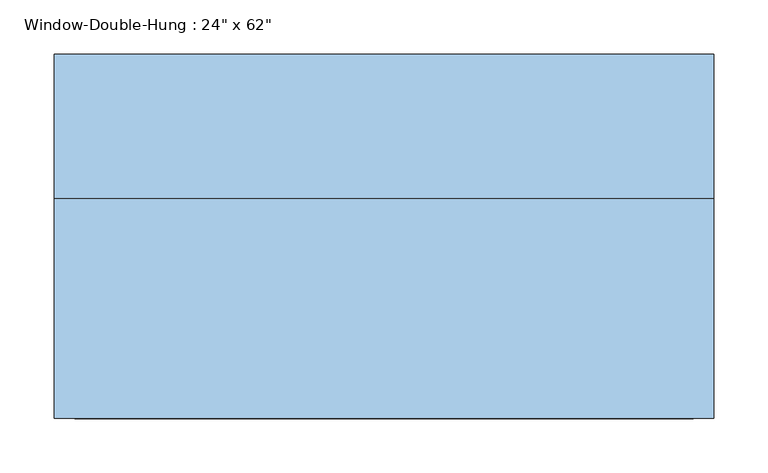
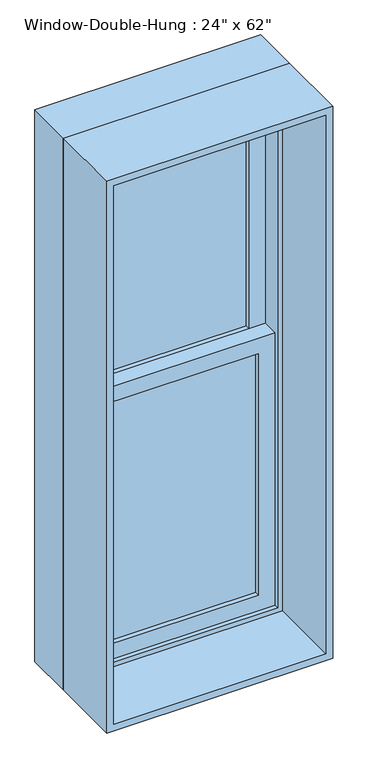
"""IFC4 building model written with IfcOpenShell, lengths in millimetres: window geometry."""

from ifc_helpers import new_model, si_unit, frame, origin, place, context, project, spatial, polyline, outline, extrude, source, transform, mapped, element, save


def window_aa90209f(model_context):
    return source(origin(), model_context, "Body", "SweptSolid", [
        extrude(outline(polyline([(228.6, 88.9), (228.6, 82.55), (-228.6, 82.55), (-228.6, 88.9), (228.6, 88.9)])), frame((0.0, 0.0, 990.6), z_axis=(0.0, 0.0, 1.0), x_axis=(1.0, 0.0, 0.0)), (0.0, 0.0, 1.0), 688.975),
        extrude(outline(polyline([(-228.6, 76.2), (228.6, 76.2), (228.6, 69.85), (-228.6, 69.85), (-228.6, 76.2)])), frame((0.0, 0.0, 990.6), z_axis=(0.0, 0.0, 1.0), x_axis=(1.0, 0.0, 0.0)), (0.0, 0.0, 1.0), 688.975),
        extrude(outline(polyline([(228.6, 133.35), (228.6, 127.0), (-228.6, 127.0), (-228.6, 133.35), (228.6, 133.35)])), frame((0.0, 0.0, 1724.025), z_axis=(0.0, 0.0, 1.0), x_axis=(1.0, 0.0, 0.0)), (0.0, 0.0, 1.0), 688.975),
        extrude(outline(polyline([(-228.6, 120.65), (228.6, 120.65), (228.6, 114.3), (-228.6, 114.3), (-228.6, 120.65)])), frame((0.0, 0.0, 1724.025), z_axis=(0.0, 0.0, 1.0), x_axis=(1.0, 0.0, 0.0)), (0.0, 0.0, 1.0), 688.975),
        extrude(outline(polyline([(1724.025, -273.05), (946.15, -273.05), (946.15, 273.05), (1724.025, 273.05), (1724.025, -273.05)]), holes=[polyline([(1679.575, 228.6), (990.6, 228.6), (990.6, -228.6), (1679.575, -228.6), (1679.575, 228.6)])]), frame((0.0, 57.15, 0.0), z_axis=(0.0, 1.0, 0.0), x_axis=(0.0, 0.0, 1.0)), (0.0, 0.0, 1.0), 44.45),
        extrude(outline(polyline([(2457.45, -273.05), (1679.575, -273.05), (1679.575, 273.05), (2457.45, 273.05), (2457.45, -273.05)]), holes=[polyline([(2413.0, 228.6), (1724.025, 228.6), (1724.025, -228.6), (2413.0, -228.6), (2413.0, 228.6)])]), frame((0.0, 101.6, 0.0), z_axis=(0.0, 1.0, 0.0), x_axis=(0.0, 0.0, 1.0)), (0.0, 0.0, 1.0), 44.45),
        extrude(outline(polyline([(2489.2, -304.8), (914.4, -304.8), (914.4, 304.8), (2489.2, 304.8), (2489.2, -304.8)]), holes=[polyline([(2457.45, 273.05), (946.15, 273.05), (946.15, -273.05), (2457.45, -273.05), (2457.45, 273.05)])]), frame((0.0, 44.45, 0.0), z_axis=(0.0, 1.0, 0.0), x_axis=(0.0, 0.0, 1.0)), (0.0, 0.0, 1.0), 133.35),
        extrude(outline(polyline([(2489.2, 304.8), (2489.2, -304.8), (914.4, -304.8), (914.4, 304.8), (2489.2, 304.8)]), holes=[polyline([(2470.15, 285.75), (933.45, 285.75), (933.45, -285.75), (2470.15, -285.75), (2470.15, 285.75)])]), frame((0.0, -158.75, 0.0), z_axis=(0.0, 1.0, 0.0), x_axis=(0.0, 0.0, 1.0)), (0.0, 0.0, 1.0), 203.2),
    ])


if __name__ == "__main__":
    model = new_model("IFC4")
    model_context = context("Model", 3, world=origin())
    ifc_project = project(units=[si_unit("LENGTHUNIT", "METRE", prefix="MILLI")], contexts=[model_context])
    site = spatial("IfcSite", under=ifc_project)
    building = spatial("IfcBuilding", under=site)
    placement = place(None, origin())
    window_shape = window_aa90209f(model_context)
    element("IfcWindow", 1, ObjectType="Window-Double-Hung : 24\" x 62\"", at=placement, inside=building, context=model_context, shape_type="MappedRepresentation", body=[
        mapped(window_shape, transform((0.0, 0.0, 0.0), x_axis=(1.0, 0.0, 0.0), y_axis=(0.0, 1.0, 0.0), z_axis=(0.0, 0.0, 1.0))),
    ])
    save(model, "model.ifc")

# Revit data of these elements
# Type "Window-Double-Hung : 24\" x 62\""
#   Type Mark = "30"
#   Fire Rating = "0.5h"
#   Construction Type Id = "DG-DR"
#   Assembly Code = "B2020100"
#   Analytic Construction = "Double glazing - domestic"
#   Wall Thickness [instance default] = 0' - 6"
#   Window Inset [instance default] = 0' - 0"
#   Visual Light Transmittance = 0.81
#   Thermal Resistance (R) = 1.8146 (h·ft²·°F)/BTU
#   Solar Heat Gain Coefficient = 0.76
#   Muntin Width = 1' - 6"
#   Muntin Height = 2' - 3 1/8"
#   Interior Wall Closure [instance default] = 0' - 1 1/2"
#   Rough Width = 2' - 0 1/2"
#   Rough Height = 5' - 2 1/2"
#   Frame Extension [instance default] = 0' - 1 1/4"
#   Exterior Wall Closure [instance default] = 0' - 0 1/2"
#   Extension Jamb [instance default] = 0' - 1 1/2"
#   Heat Transfer Coefficient (U) = 0.5511 BTU/(h·ft²·°F)
#   Height = 5' - 2"
#   Width = 2' - 0"
#   Top Muntin Visibility = yes
#   Indicator Visibility [instance default] = yes
#   Extension Jamb Visibility [instance default] = yes
#   Interior Trim Visibility [instance default] = yes
#   Exterior Trim Visibility [instance default] = yes
#   Define Thermal Properties by = 1
#   Bottom Muntin Visibility = yes
#   Muntin Pattern = Muntin Pattern_2x2 : Muntin Pattern_2x2
#   Interior Trim Material = Wood - Stained
#   Interior Trim = Trim-Window-Interior-Flat : Picture Frame
#   Exterior Trim Material = Clad - White
#   Exterior Trim = Trim-Window-Exterior-Flat : with Sill
#   Glass Panel Material = Glass
#   Exterior Frame Material = Clad - White
#   Interior Frame Material = Wood - Stained
#   Wall Closure = (empty or 0)
# Element 1 (IfcWindow, "Window-Double-Hung : 24\" x 62\"")
#   Wall Thickness = 1' - 0 1/2"
#   Extension Jamb = 0' - 8"
#   Materials on its faces: "Wood - Stained", "Glass", "Clad - White"
# Materials
#   "Wood - Stained": class "Wood", colour RGB 224 178 126, transparency 0, Cost = 0
#   "Clad - White": class "Wood", colour RGB 242 242 238, transparency 0, Cost = 0
#   "Glass": class "Glass", colour RGB 0 128 192, transparency 0.75, Description = "Soda Lime Glass", Cost = 0
